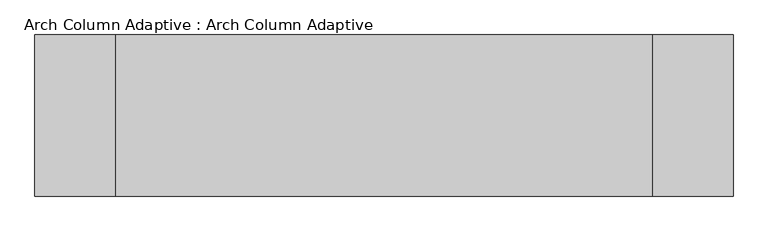
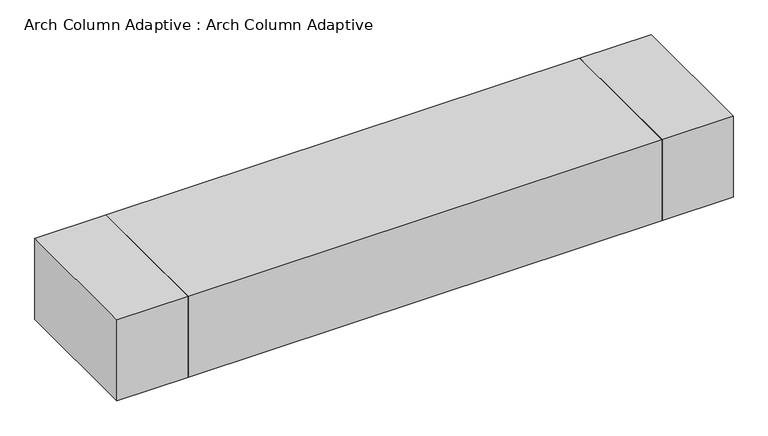
"""IFC4 building model written with IfcOpenShell, lengths in millimetres: proxy geometry, Arch Column Adaptive : Arch Column Adaptive."""

import ifcopenshell
import ifcopenshell.guid

model = None  # the IFC model being written
_history = None  # IfcOwnerHistory: only IFC2X3 demands one
_inside = {}  # id of a spatial element -> (the spatial element, [elements in it])
_under = {}  # id of a project, library or spatial element -> (it, [spatial elements below it])
_declared = {}  # id of a project -> (the project, [libraries it declares])
_typed = {}  # id of a type object -> (the type object, [elements of that type])
_made_of = {}  # id of a material, layer set ... -> (it, [elements and type objects made of it])


def new_model(schema):
    """Start an empty IFC model of exactly this schema.

    Asked for "IFC4X3", IfcOpenShell would pick the latest addendum, in which some entities
    have other attributes; the version numbers below select the first issue.
    IFC2X3 requires an IfcOwnerHistory on every rooted entity: one is made here for all.
    """
    global model, _history
    if schema == "IFC4X3":
        model = ifcopenshell.file(schema_version=(4, 3, 0, 0))
    else:
        model = ifcopenshell.file(schema=schema)
    _inside.clear()
    _under.clear()
    _declared.clear()
    _typed.clear()
    _made_of.clear()
    _history = None
    if model.schema == "IFC2X3":
        org = make("IfcOrganization", Name="unknown")
        user = make(
            "IfcPersonAndOrganization",
            ThePerson=make("IfcPerson", FamilyName="unknown"),
            TheOrganization=org,
        )
        app = make(
            "IfcApplication",
            ApplicationDeveloper=org,
            Version="unknown",
            ApplicationFullName="unknown",
            ApplicationIdentifier="unknown",
        )
        _history = make(
            "IfcOwnerHistory",
            OwningUser=user,
            OwningApplication=app,
            ChangeAction="ADDED",
            CreationDate=0,
        )
    return model


def make(cls, **values):
    """One entity of the class cls with the attributes given. An attribute that is None is left unset."""
    return model.create_entity(
        cls, **{name: value for name, value in values.items() if value is not None}
    )


def rooted(cls, **values):
    """An entity with a GlobalId (a new one), such as an element, a storey or a relation."""
    return make(cls, GlobalId=ifcopenshell.guid.new(), OwnerHistory=_history, **values)


def si_unit(unit_type, name, prefix=None):
    """IfcSIUnit, for example si_unit("LENGTHUNIT", "METRE", prefix="MILLI")."""
    return make("IfcSIUnit", UnitType=unit_type, Prefix=prefix, Name=name)


def assignment(units):
    """IfcUnitAssignment: the units of a project."""
    return None if units is None else make("IfcUnitAssignment", Units=units)


def point(xyz):
    """IfcCartesianPoint."""
    return None if xyz is None else make("IfcCartesianPoint", Coordinates=xyz)


def direction(xyz):
    """IfcDirection."""
    return None if xyz is None else make("IfcDirection", DirectionRatios=xyz)


def frame(location, z_axis=None, x_axis=None):
    """IfcAxis2Placement3D, a coordinate frame: its origin and axes. An axis left out is left unset."""
    return make(
        "IfcAxis2Placement3D",
        Location=point(location),
        Axis=direction(z_axis),
        RefDirection=direction(x_axis),
    )


def origin():
    """The frame at (0, 0, 0) with its axes left unset."""
    return frame((0.0, 0.0, 0.0))


def place(relative_to, where):
    """IfcLocalPlacement: puts the frame where relative to a parent placement (None: the world)."""
    return make(
        "IfcLocalPlacement", PlacementRelTo=relative_to, RelativePlacement=where
    )


def context(
    kind, dimensions, precision=None, world=None, true_north=None, identifier=None
):
    """IfcGeometricRepresentationContext, for example the 3D "Model" context."""
    return make(
        "IfcGeometricRepresentationContext",
        ContextIdentifier=identifier,
        ContextType=kind,
        CoordinateSpaceDimension=dimensions,
        Precision=precision,
        WorldCoordinateSystem=world,
        TrueNorth=true_north,
    )


def project(units=None, contexts=None):
    """IfcProject with its units and contexts."""
    return rooted(
        "IfcProject",
        Name="project",
        RepresentationContexts=contexts,
        UnitsInContext=assignment(units),
    )


def spatial(cls, under=None, at=None, **own):
    """A site, building, storey or space (cls), placed at a placement, below another one or the project."""
    s = rooted(cls, ObjectPlacement=at, **own)
    if under is not None:
        _under.setdefault(under.id(), (under, []))[1].append(s)
    return s


def polyline(points):
    """IfcPolyline through the points."""
    return make("IfcPolyline", Points=[point(p) for p in points])


def outline(outer, holes=None, kind="AREA"):
    """IfcArbitraryClosedProfileDef: a profile drawn as a closed curve; with holes, ...WithVoids."""
    if holes is None:
        return make("IfcArbitraryClosedProfileDef", ProfileType=kind, OuterCurve=outer)
    return make(
        "IfcArbitraryProfileDefWithVoids",
        ProfileType=kind,
        OuterCurve=outer,
        InnerCurves=holes,
    )


def extrude(swept, where, along, depth):
    """IfcExtrudedAreaSolid: the profile swept, set in the frame where, extruded along a direction by depth."""
    return make(
        "IfcExtrudedAreaSolid",
        SweptArea=swept,
        Position=where,
        ExtrudedDirection=direction(along),
        Depth=depth,
    )


def shape(context_of_items, identifier, shape_type, items):
    """IfcShapeRepresentation: the items that make up one representation, for example the "Body"."""
    return make(
        "IfcShapeRepresentation",
        ContextOfItems=context_of_items,
        RepresentationIdentifier=identifier,
        RepresentationType=shape_type,
        Items=items,
    )


def source(mapping_origin, context_of_items, identifier, shape_type, items):
    """IfcRepresentationMap: a shape defined once, which mapped items show again and again."""
    return make(
        "IfcRepresentationMap",
        MappingOrigin=mapping_origin,
        MappedRepresentation=shape(context_of_items, identifier, shape_type, items),
    )


def transform(
    local_origin,
    x_axis=None,
    y_axis=None,
    z_axis=None,
    scale=None,
    scale2=None,
    scale3=None,
    uniform=True,
):
    """IfcCartesianTransformationOperator3D, or its non-uniform kind. x_axis, y_axis, z_axis: its Axis1, 2, 3."""
    if uniform:
        return make(
            "IfcCartesianTransformationOperator3D",
            Axis1=direction(x_axis),
            Axis2=direction(y_axis),
            LocalOrigin=point(local_origin),
            Scale=scale,
            Axis3=direction(z_axis),
        )
    return make(
        "IfcCartesianTransformationOperator3DnonUniform",
        Axis1=direction(x_axis),
        Axis2=direction(y_axis),
        LocalOrigin=point(local_origin),
        Scale=scale,
        Axis3=direction(z_axis),
        Scale2=scale2,
        Scale3=scale3,
    )


def mapped(mapping_source, mapping_target):
    """IfcMappedItem: shows the shape of a source again, moved by a transform."""
    return make(
        "IfcMappedItem", MappingSource=mapping_source, MappingTarget=mapping_target
    )


def made_of(thing, what):
    """Note that an element or type object is made of a material, layer set ...; save() writes the relation."""
    if what is not None:
        _made_of.setdefault(what.id(), (what, []))[1].append(thing)
    return thing


def element(
    cls,
    number,
    at=None,
    inside=None,
    cuts=None,
    type_object=None,
    material=None,
    context=None,
    identifier="Body",
    shape_type=None,
    held_by="IfcProductDefinitionShape",
    body=None,
    shapes=None,
    **own,
):
    """One element of the class cls, such as IfcWall. Its Tag is "e" and its number.

    at: its placement. inside: the storey or other place that contains it. cuts: it is an
    opening in that element (IfcRelVoidsElement). A single representation is given by context,
    identifier, shape_type and body (its items); several are given by shapes. held_by: the class
    of the entity that holds the representations. save() writes the other relations.
    """
    e = rooted(cls, Tag="e%d" % number, ObjectPlacement=at, **own)
    if body is not None:
        shapes = [shape(context, identifier, shape_type, body)]
    if shapes is not None:
        e.Representation = make(held_by, Representations=shapes)
    if inside is not None:
        _inside.setdefault(inside.id(), (inside, []))[1].append(e)
    if cuts is not None:
        rooted(
            "IfcRelVoidsElement", RelatingBuildingElement=cuts, RelatedOpeningElement=e
        )
    if type_object is not None:
        _typed.setdefault(type_object.id(), (type_object, []))[1].append(e)
    return made_of(e, material)


def aggregate(whole, parts):
    """IfcRelAggregates: a whole, such as a stair, and the parts it consists of."""
    return rooted("IfcRelAggregates", RelatingObject=whole, RelatedObjects=parts)


def save(model, path):
    """Write the relations noted so far, then the file.

    IfcRelAggregates (storeys below a building ...), IfcRelContainedInSpatialStructure (elements
    in a storey), IfcRelDefinesByType, IfcRelAssociatesMaterial and IfcRelDeclares: one each for
    every whole, place, type object, material and project.
    """
    for whole, parts in _under.values():
        aggregate(whole, parts)
    for where, things in _inside.values():
        rooted(
            "IfcRelContainedInSpatialStructure",
            RelatedElements=things,
            RelatingStructure=where,
        )
    for kind, things in _typed.values():
        rooted("IfcRelDefinesByType", RelatedObjects=things, RelatingType=kind)
    for what, things in _made_of.values():
        rooted("IfcRelAssociatesMaterial", RelatedObjects=things, RelatingMaterial=what)
    for by, libraries in _declared.values():
        rooted("IfcRelDeclares", RelatingContext=by, RelatedDefinitions=libraries)
    model.write(path)


def arch_column_adaptive_arch_column_adaptive_9be84d25(model_context):
    return source(origin(), model_context, "Body", "SweptSolid", [
        extrude(outline(polyline([(5000.0, -1500.0), (5000.0, 1500.0), (6500.0, 1500.0), (6500.0, -1500.0), (5000.0, -1500.0)])), frame((0.0, 0.0, 79290.0), z_axis=(0.0, 0.0, 1.0), x_axis=(1.0, 0.0, 0.0)), (0.0, 0.0, 1.0), 1800.0),
        extrude(outline(polyline([(-5000.0, 1500.0), (-5000.0, -1500.0), (-6500.0, -1500.0), (-6500.0, 1500.0), (-5000.0, 1500.0)])), frame((0.0, 0.0, 79290.0), z_axis=(0.0, 0.0, 1.0), x_axis=(1.0, 0.0, 0.0)), (0.0, 0.0, 1.0), 1800.0),
        extrude(outline(polyline([(-5000.0, -1500.0), (-5000.0, 1500.0), (5000.0, 1500.0), (5000.0, -1500.0), (-5000.0, -1500.0)])), frame((0.0, 0.0, 79290.0), z_axis=(0.0, 0.0, 1.0), x_axis=(1.0, 0.0, 0.0)), (0.0, 0.0, 1.0), 1800.0),
    ])


if __name__ == "__main__":
    model = new_model("IFC4")
    model_context = context("Model", 3, world=origin())
    ifc_project = project(units=[si_unit("LENGTHUNIT", "METRE", prefix="MILLI")], contexts=[model_context])
    site = spatial("IfcSite", under=ifc_project)
    building = spatial("IfcBuilding", under=site)
    placement = place(None, origin())
    arch_column_adaptive_arch_column_adaptive_shape = arch_column_adaptive_arch_column_adaptive_9be84d25(model_context)
    element("IfcBuildingElementProxy", 1, Name="Arch Column Adaptive : Arch Column Adaptive", ObjectType="Arch Column Adaptive : Arch Column Adaptive", at=placement, inside=building, context=model_context, shape_type="MappedRepresentation", body=[
        mapped(arch_column_adaptive_arch_column_adaptive_shape, transform((0.0, 0.0, 0.0), x_axis=(1.0, 0.0, 0.0), y_axis=(0.0, 1.0, 0.0), z_axis=(0.0, 0.0, 1.0))),
    ])
    save(model, "model.ifc")

# Revit data of these elements
# Type "Arch Column Adaptive : Arch Column Adaptive"
#   Top Width = 3000 mm
#   Length [instance default] = 21000 mm
#   Height [instance default] = 50000 mm
#   Default Elevation = 0
# Element 1 (IfcBuildingElementProxy, "Arch Column Adaptive : Arch Column Adaptive")
#   Height = 79290 mm
